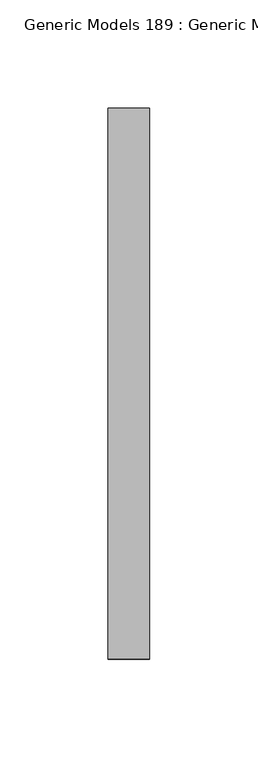
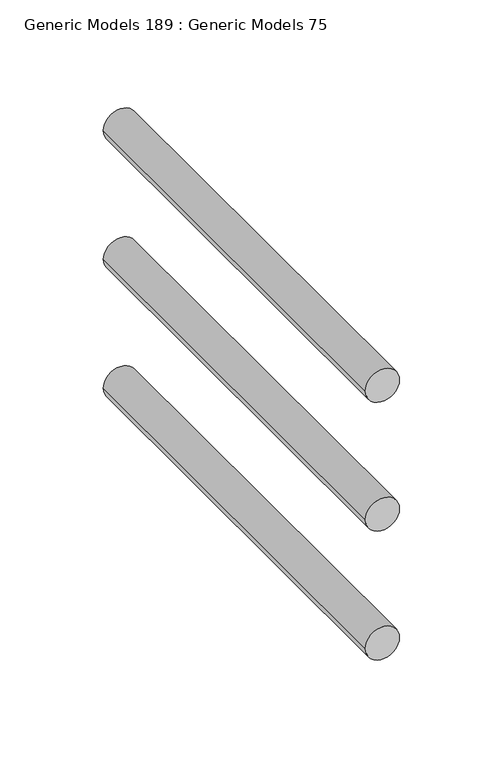
"""IFC4 building model written with IfcOpenShell, lengths in millimetres: proxy geometry, Generic Models 189 : Generic Models 75."""

from ifc_helpers import new_model, si_unit, point, frame, frame_2d, origin, place, context, project, spatial, circle_curve, trimmed, segment, composite_curve, outline, extrude, source, transform, mapped, element, save


def generic_models_189_generic_models_75_b51f780d(model_context):
    return source(origin(), model_context, "Body", "SweptSolid", [
        extrude(outline(composite_curve([segment(trimmed(circle_curve(frame_2d((268976.475, 31705.5346032)), 9.525), [point((268976.475, 31696.0096032))], [point((268976.475, 31715.0596032))], False, "CARTESIAN"), True, "CONTINUOUS"), segment(trimmed(circle_curve(frame_2d((268976.475, 31705.5346032)), 9.525), [point((268976.475, 31715.0596032))], [point((268976.475, 31696.0096032))], False, "CARTESIAN"), True, "CONTINUOUS")], self_intersect=False)), frame((0.0, 30647.3406612, 0.0), z_axis=(0.0, 1.0, 0.0), x_axis=(0.0, 0.0, 1.0)), (0.0, 0.0, 1.0), 254.0),
        extrude(outline(composite_curve([segment(trimmed(circle_curve(frame_2d((268900.275, 31705.5346032)), 9.525), [point((268900.275, 31696.0096032))], [point((268900.275, 31715.0596032))], False, "CARTESIAN"), True, "CONTINUOUS"), segment(trimmed(circle_curve(frame_2d((268900.275, 31705.5346032)), 9.525), [point((268900.275, 31715.0596032))], [point((268900.275, 31696.0096032))], False, "CARTESIAN"), True, "CONTINUOUS")], self_intersect=False)), frame((0.0, 30647.3406612, 0.0), z_axis=(0.0, 1.0, 0.0), x_axis=(0.0, 0.0, 1.0)), (0.0, 0.0, 1.0), 254.0),
        extrude(outline(composite_curve([segment(trimmed(circle_curve(frame_2d((269052.675, 31705.5346032)), 9.525), [point((269052.675, 31696.0096032))], [point((269052.675, 31715.0596032))], False, "CARTESIAN"), True, "CONTINUOUS"), segment(trimmed(circle_curve(frame_2d((269052.675, 31705.5346032)), 9.525), [point((269052.675, 31715.0596032))], [point((269052.675, 31696.0096032))], False, "CARTESIAN"), True, "CONTINUOUS")], self_intersect=False)), frame((0.0, 30647.3406612, 0.0), z_axis=(0.0, 1.0, 0.0), x_axis=(0.0, 0.0, 1.0)), (0.0, 0.0, 1.0), 254.0),
    ])


if __name__ == "__main__":
    model = new_model("IFC4")
    model_context = context("Model", 3, world=origin())
    ifc_project = project(units=[si_unit("LENGTHUNIT", "METRE", prefix="MILLI")], contexts=[model_context])
    site = spatial("IfcSite", under=ifc_project)
    building = spatial("IfcBuilding", under=site)
    placement = place(None, origin())
    generic_models_189_generic_models_75_shape = generic_models_189_generic_models_75_b51f780d(model_context)
    element("IfcBuildingElementProxy", 1, Name="Generic Models 189 : Generic Models 75", ObjectType="Generic Models 189 : Generic Models 75", at=placement, inside=building, context=model_context, shape_type="MappedRepresentation", body=[
        mapped(generic_models_189_generic_models_75_shape, transform((0.0, 0.0, 0.0), x_axis=(1.0, 0.0, 0.0), y_axis=(0.0, 1.0, 0.0), z_axis=(0.0, 0.0, 1.0))),
    ])
    save(model, "model.ifc")
